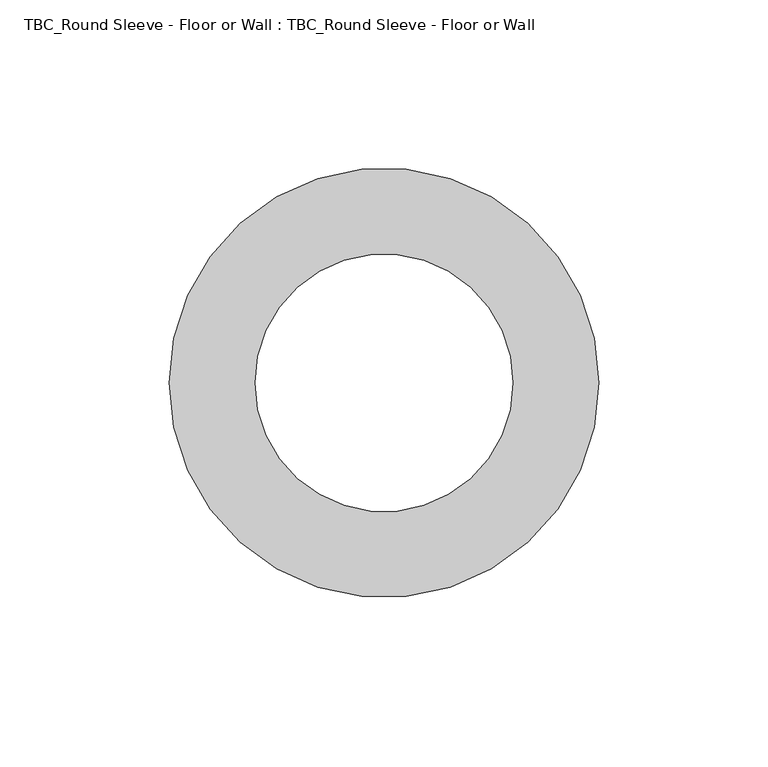
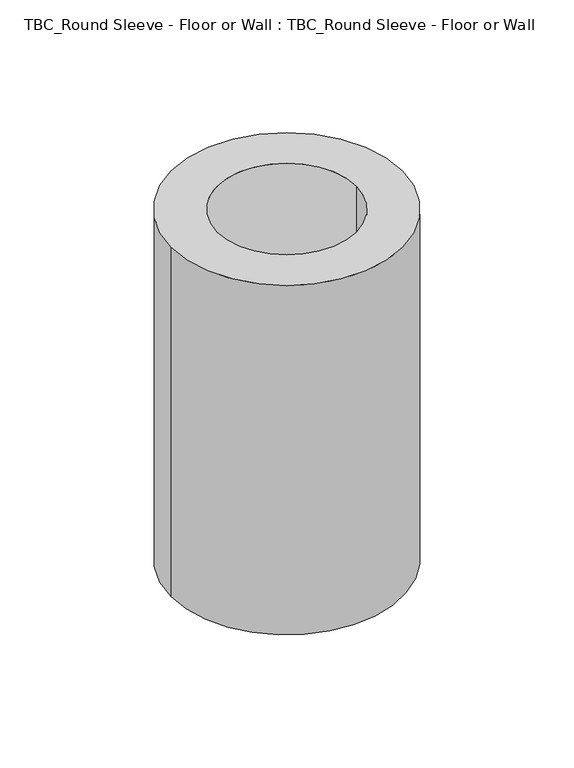
"""IFC4 building model written with IfcOpenShell, lengths in millimetres: proxy geometry, TBC_Round Sleeve - Floor or Wall : TBC_Round Sleeve - Floor or Wall."""

from ifc_helpers import new_model, si_unit, point, frame, origin, origin_2d, place, context, project, spatial, circle_curve, trimmed, segment, composite_curve, outline, extrude, source, transform, mapped, element, save


def tbc_round_sleeve_floor_or_wall_tbc_round_sleeve_floor_or_bcb517f5(model_context):
    return source(origin(), model_context, "Body", "SweptSolid", [
        extrude(outline(composite_curve([segment(trimmed(circle_curve(origin_2d(), 63.5), [point((-63.5, 0.0))], [point((63.5, 0.0))], False, "CARTESIAN"), True, "CONTINUOUS"), segment(trimmed(circle_curve(origin_2d(), 63.5), [point((63.5, 0.0))], [point((-63.5, 0.0))], False, "CARTESIAN"), True, "CONTINUOUS")], self_intersect=False), holes=[composite_curve([segment(trimmed(circle_curve(origin_2d(), 38.1), [point((-38.1, 0.0))], [point((38.1, 0.0))], True, "CARTESIAN"), True, "CONTINUOUS"), segment(trimmed(circle_curve(origin_2d(), 38.1), [point((38.1, 0.0))], [point((-38.1, 0.0))], True, "CARTESIAN"), True, "CONTINUOUS")], self_intersect=False)]), frame((0.0, 0.0, -203.2), z_axis=(0.0, 0.0, 1.0), x_axis=(1.0, 0.0, 0.0)), (0.0, 0.0, 1.0), 203.2),
    ])


if __name__ == "__main__":
    model = new_model("IFC4")
    model_context = context("Model", 3, world=origin())
    ifc_project = project(units=[si_unit("LENGTHUNIT", "METRE", prefix="MILLI")], contexts=[model_context])
    site = spatial("IfcSite", under=ifc_project)
    building = spatial("IfcBuilding", under=site)
    placement = place(None, origin())
    tbc_round_sleeve_floor_or_wall_tbc_round_sleeve_floor_or_shape = tbc_round_sleeve_floor_or_wall_tbc_round_sleeve_floor_or_bcb517f5(model_context)
    element("IfcBuildingElementProxy", 1, Name="TBC_Round Sleeve - Floor or Wall : TBC_Round Sleeve - Floor or Wall", ObjectType="TBC_Round Sleeve - Floor or Wall : TBC_Round Sleeve - Floor or Wall", at=placement, inside=building, context=model_context, shape_type="MappedRepresentation", body=[
        mapped(tbc_round_sleeve_floor_or_wall_tbc_round_sleeve_floor_or_shape, transform((0.0, 0.0, 0.0), x_axis=(1.0, 0.0, 0.0), y_axis=(0.0, 1.0, 0.0), z_axis=(0.0, 0.0, 1.0))),
    ])
    save(model, "model.ifc")

# Revit data of these elements
# Type "TBC_Round Sleeve - Floor or Wall : TBC_Round Sleeve - Floor or Wall"
#   Tag Dimension [instance default] = ""
#   MEP Type [instance default] = ""
#   MEP Element [instance default] = ""
#   MEP Category [instance default] = ""
#   Host Element Type [instance default] = ""
#   Host Element Id [instance default] = ""
#   Host Element Category [instance default] = ""
#   Control Line Y [instance default] = ""
#   Control Line X [instance default] = ""
#   Sleeve Radius [instance default] = 1' - 0"
#   Sleeve Edge [instance default] = 1' - 2"
#   Sleeve Depth [instance default] = 3' - 0"
#   Distance Y [instance default] = 0' - 0"
#   Distance X [instance default] = 0' - 0"
#   Default Elevation = 0
# Element 1 (IfcBuildingElementProxy, "TBC_Round Sleeve - Floor or Wall : TBC_Round Sleeve - Floor or Wall")
#   Tag Dimension = "5\"ø"
#   MEP Type = "PLG-S"
#   MEP Element = "1027799"
#   MEP Category = "Pipe"
#   Host Element Type = "8\" Plank"
#   Host Element Id = "529506"
#   Host Element Category = "Floors"
#   Sleeve Radius = 0' - 3"
#   Sleeve Edge = 0' - 5"
#   Sleeve Depth = 0' - 8"
